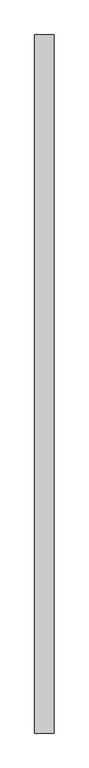
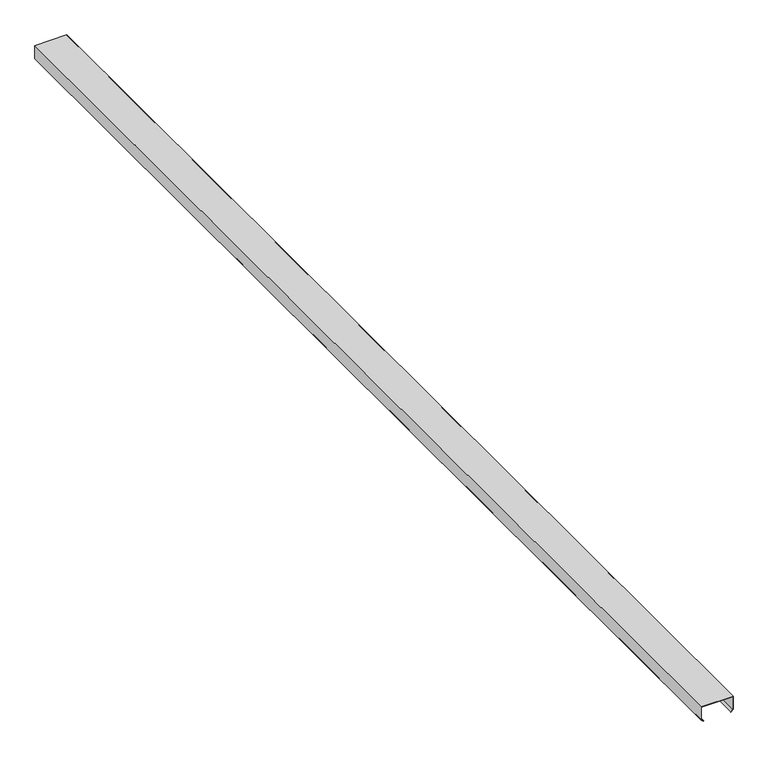
"""IFC4 building model written with IfcOpenShell, lengths in millimetres: proxy geometry, Generic Models 7:Generic Models 1:1:Generic Models 1:1 : Generic Models 7:Generic Models 1:337419:22 : Generic Models 7:Generic Models 1:1:Generic Models 1:1 : Generic Models 7:Generic Models 1:337419:306201."""

from ifc_helpers import new_model, si_unit, frame, origin, place, context, project, spatial, polyline, outline, extrude, source, transform, mapped, element, save


def generic_models_2511116c(model_context):
    return source(origin(), model_context, "Body", "SweptSolid", [
        extrude(outline(polyline([(4985.940625, 560556.1617239), (4985.940625, 560352.9617239), (4897.040625, 560352.9617239), (4884.7955211, 560367.5548705), (4886.9236883, 560369.3406148), (4898.336086, 560355.7398489), (4983.1625, 560355.7398489), (4983.1625, 560553.3835989), (4898.336086, 560553.3835989), (4886.9236883, 560539.7828329), (4884.7955211, 560541.5685772), (4897.040625, 560556.1617239), (4985.940625, 560556.1617239)])), frame((0.0, -579000.6913841, 0.0), z_axis=(0.0, 1.0, 0.0), x_axis=(0.0, 0.0, 1.0)), (0.0, 0.0, 1.0), 7315.2),
    ])


if __name__ == "__main__":
    model = new_model("IFC4")
    model_context = context("Model", 3, world=origin())
    ifc_project = project(units=[si_unit("LENGTHUNIT", "METRE", prefix="MILLI")], contexts=[model_context])
    site = spatial("IfcSite", under=ifc_project)
    building = spatial("IfcBuilding", under=site)
    placement = place(None, origin())
    generic_models_shape = generic_models_2511116c(model_context)
    element("IfcBuildingElementProxy", 1, Name="Generic Models 7:Generic Models 1:1:Generic Models 1:1 : Generic Models 7:Generic Models 1:337419:22 : Generic Models 7:Generic Models 1:1:Generic Models 1:1 : Generic Models 7:Generic Models 1:337419:306201", ObjectType="Generic Models 7:Generic Models 1:1:Generic Models 1:1 : Generic Models 7:Generic Models 1:337419:22 : Generic Models 7:Generic Models 1:1:Generic Models 1:1 : Generic Models 7:Generic Models 1:337419:306201", at=placement, inside=building, context=model_context, shape_type="MappedRepresentation", body=[
        mapped(generic_models_shape, transform((0.0, 0.0, 0.0), x_axis=(1.0, 0.0, 0.0), y_axis=(0.0, 1.0, 0.0), z_axis=(0.0, 0.0, 1.0))),
    ])
    save(model, "model.ifc")

# Revit data of these elements
# Type "Generic Models 7:Generic Models 1:1:Generic Models 1:1 : Generic Models 7:Generic Models 1:337419:22 : Generic Models 7:Generic Models 1:1:Generic Models 1:1 : Generic Models 7:Generic Models 1:337419:306201"
#   NameOverride = "Generic Models 7:Generic Models 1:1:Generic Models 1:1 : Generic Models 7:Generic Models 1:337419:306201"
#   ObjectTypeOverride = "Generic Models 1:1 : Generic Models 7:Generic Models 1:337419"
#   Reference = "Generic Models 1"
#   Tag = "306201"
# Element 1 (IfcBuildingElementProxy, "Generic Models 7:Generic Models 1:1:Generic Models 1:1 : Generic Models 7:Generic Models 1:337419:22 : Generic Models 7:Generic Models 1:1:Generic Models 1:1 : Generic Models 7:Generic Models 1:337419:306201")
#   Materials on its faces: "CEE' SECTION (8.0x3.5C - SEE STRUCT. DWGS)"
# Materials
#   "CEE' SECTION (8.0x3.5C - SEE STRUCT. DWGS)": class "Unassigned", colour RGB 210 209 208, transparency 0, Keynote = "M05121300.02", Cost = 0
